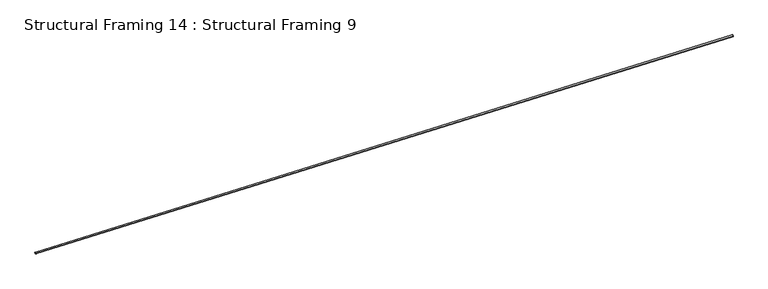
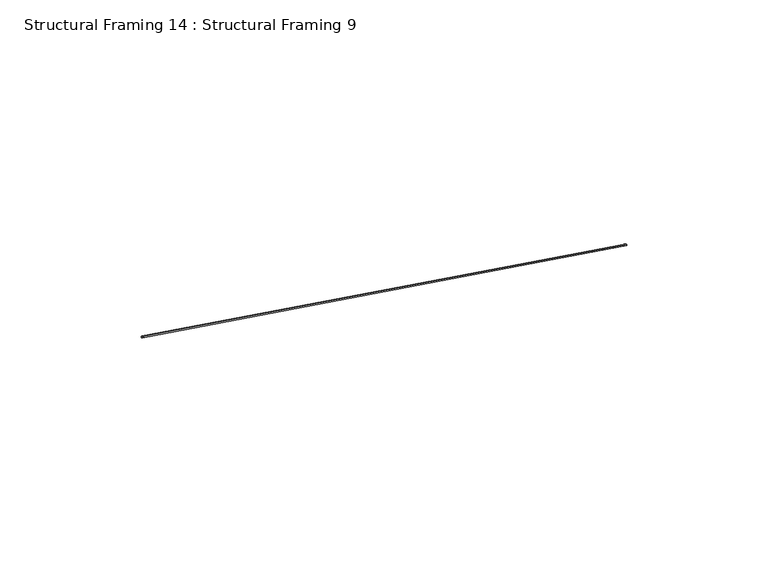
"""IFC4 building model written with IfcOpenShell, lengths in millimetres: beam geometry, Structural Framing 14 : Structural Framing 9."""

from ifc_helpers import new_model, si_unit, point, frame, origin, origin_2d, place, context, project, spatial, circle_curve, trimmed, segment, composite_curve, outline, extrude, source, transform, mapped, element, save


def structural_framing_14_structural_framing_9_291d0cf0(model_context):
    return source(origin(), model_context, "Body", "SweptSolid", [
        extrude(outline(composite_curve([segment(trimmed(circle_curve(origin_2d(), 6.35), [point((0.0, -6.35))], [point((0.0, 6.35))], False, "CARTESIAN"), True, "CONTINUOUS"), segment(trimmed(circle_curve(origin_2d(), 6.35), [point((0.0, 6.35))], [point((0.0, -6.35))], False, "CARTESIAN"), True, "CONTINUOUS")], self_intersect=False)), frame((17936.6160052, 11688.3780277, 2959.3363832), z_axis=(-0.8989286779363542, -0.28046158673269656, 0.33655390407923746), x_axis=(0.0, -0.7682212795973775, -0.6401843996644778)), (0.0, 0.0, 1.0), 5845.7129347),
    ])


if __name__ == "__main__":
    model = new_model("IFC4")
    model_context = context("Model", 3, world=origin())
    ifc_project = project(units=[si_unit("LENGTHUNIT", "METRE", prefix="MILLI")], contexts=[model_context])
    site = spatial("IfcSite", under=ifc_project)
    building = spatial("IfcBuilding", under=site)
    placement = place(None, origin())
    structural_framing_14_structural_framing_9_shape = structural_framing_14_structural_framing_9_291d0cf0(model_context)
    element("IfcBeam", 1, ObjectType="Structural Framing 14 : Structural Framing 9", at=placement, inside=building, context=model_context, shape_type="MappedRepresentation", body=[
        mapped(structural_framing_14_structural_framing_9_shape, transform((0.0, 0.0, 0.0), x_axis=(1.0, 0.0, 0.0), y_axis=(0.0, 1.0, 0.0), z_axis=(0.0, 0.0, 1.0))),
    ])
    save(model, "model.ifc")

# Revit data of these elements
# Type "Structural Framing 14 : Structural Framing 9"
#   Structural Material [instance default] = EXISTING LATERAL BRACING (1/4" CABLE)
# Element 1 (IfcBeam, "Structural Framing 14 : Structural Framing 9")
#   Materials on its faces: "EXISTING LATERAL BRACING (1/4\" CABLE)"
# Materials
#   "EXISTING LATERAL BRACING (1/4\" CABLE)": class "Generic", colour RGB 120 120 120, transparency 0, Cost = 0
